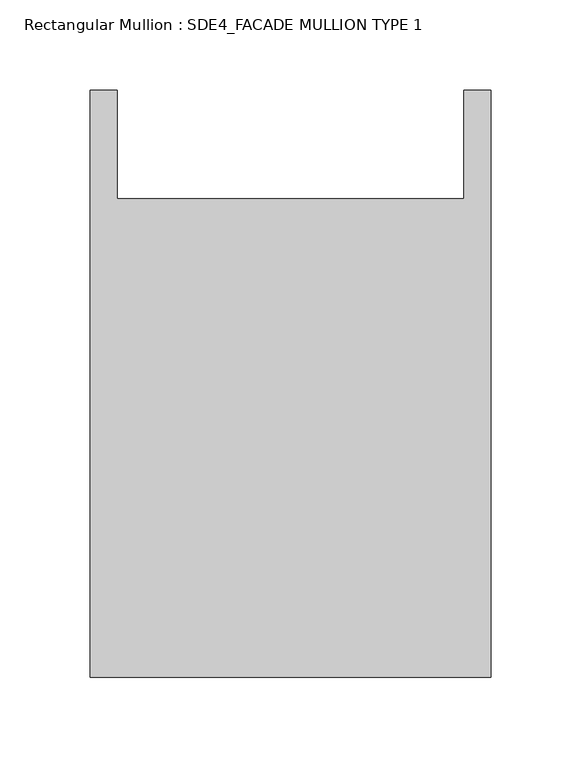
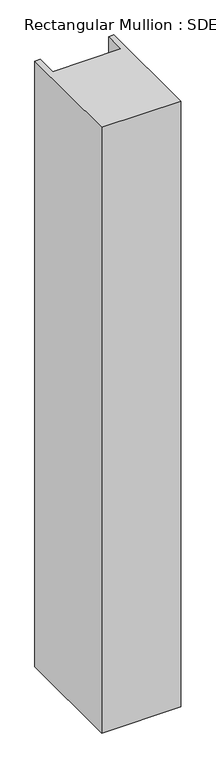
"""IFC4 building model written with IfcOpenShell, lengths in millimetres: member geometry, Rectangular Mullion : SDE4_FACADE MULLION TYPE 1."""

from ifc_helpers import new_model, si_unit, frame, origin, place, context, project, spatial, polyline, outline, extrude, source, transform, mapped, element, save


def rectangular_mullion_sde4_facade_mullion_type_1_b45dacb8(model_context):
    return source(origin(), model_context, "Body", "SweptSolid", [
        extrude(outline(polyline([(111.0, -132.5), (-111.0, -132.5), (-111.0, 192.5), (-96.0, 192.5), (-96.0, 132.5), (96.0, 132.5), (96.0, 192.5), (111.0, 192.5), (111.0, -132.5)])), frame((0.0, 0.0, -1800.0), z_axis=(0.0, 0.0, 1.0), x_axis=(1.0, 0.0, 0.0)), (0.0, 0.0, 1.0), 1800.0),
    ])


if __name__ == "__main__":
    model = new_model("IFC4")
    model_context = context("Model", 3, world=origin())
    ifc_project = project(units=[si_unit("LENGTHUNIT", "METRE", prefix="MILLI")], contexts=[model_context])
    site = spatial("IfcSite", under=ifc_project)
    building = spatial("IfcBuilding", under=site)
    placement = place(None, origin())
    rectangular_mullion_sde4_facade_mullion_type_1_shape = rectangular_mullion_sde4_facade_mullion_type_1_b45dacb8(model_context)
    element("IfcMember", 1, ObjectType="Rectangular Mullion : SDE4_FACADE MULLION TYPE 1", at=placement, inside=building, context=model_context, shape_type="MappedRepresentation", body=[
        mapped(rectangular_mullion_sde4_facade_mullion_type_1_shape, transform((0.0, 0.0, 0.0), x_axis=(1.0, 0.0, 0.0), y_axis=(0.0, 1.0, 0.0), z_axis=(0.0, 0.0, 1.0))),
    ])
    save(model, "model.ifc")

# Revit data of these elements
# Type "Rectangular Mullion : SDE4_FACADE MULLION TYPE 1"
#   built-in parameter 1007322 = 0.869423 (stored number, unit not read)
#   built-in parameter 1007321 = 0.364173 (stored number, unit not read)
#   built-in parameter 1007320 = 0.364173 (stored number, unit not read)
